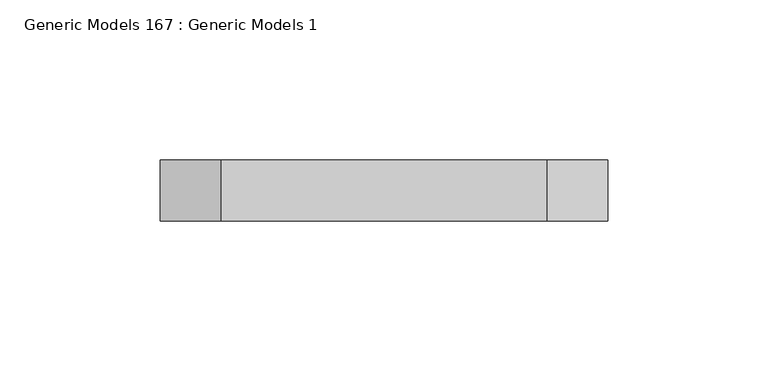
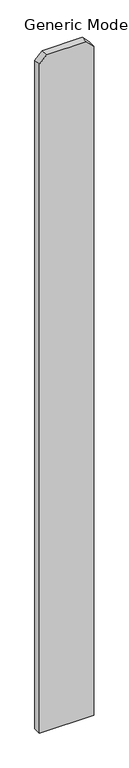
"""IFC4 building model written with IfcOpenShell, lengths in millimetres: proxy geometry, Generic Models 167 : Generic Models 1."""

from ifc_helpers import new_model, si_unit, frame, origin, place, context, project, spatial, polyline, outline, extrude, source, transform, mapped, element, save


def generic_models_167_generic_models_1_3792af48(model_context):
    return source(origin(), model_context, "Body", "SweptSolid", [
        extrude(outline(polyline([(76.2, 55446.6125), (1885.95, 55446.6125), (1905.0, 55427.5625), (1905.0, 55325.9625), (1885.95, 55306.9125), (76.2, 55306.9125), (76.2, 55446.6125)])), frame((0.0, 547.6875, 0.0), z_axis=(0.0, 1.0, 0.0), x_axis=(0.0, 0.0, 1.0)), (0.0, 0.0, 1.0), 19.05),
    ])


if __name__ == "__main__":
    model = new_model("IFC4")
    model_context = context("Model", 3, world=origin())
    ifc_project = project(units=[si_unit("LENGTHUNIT", "METRE", prefix="MILLI")], contexts=[model_context])
    site = spatial("IfcSite", under=ifc_project)
    building = spatial("IfcBuilding", under=site)
    placement = place(None, origin())
    generic_models_167_generic_models_1_shape = generic_models_167_generic_models_1_3792af48(model_context)
    element("IfcBuildingElementProxy", 1, Name="Generic Models 167 : Generic Models 1", ObjectType="Generic Models 167 : Generic Models 1", at=placement, inside=building, context=model_context, shape_type="MappedRepresentation", body=[
        mapped(generic_models_167_generic_models_1_shape, transform((0.0, 0.0, 0.0), x_axis=(1.0, 0.0, 0.0), y_axis=(0.0, 1.0, 0.0), z_axis=(0.0, 0.0, 1.0))),
    ])
    save(model, "model.ifc")

# Revit data of these elements
# Element 1 (IfcBuildingElementProxy, "Generic Models 167 : Generic Models 1")
#   Materials on its faces: "VERTICAL 1X6 CEDAR PLANKS W/ CLEAR WOOD SEALER"
# Materials
#   "VERTICAL 1X6 CEDAR PLANKS W/ CLEAR WOOD SEALER": class "Wood", colour RGB 234 198 147, transparency 0, Description = "Pinus Echinata", Cost = 0
